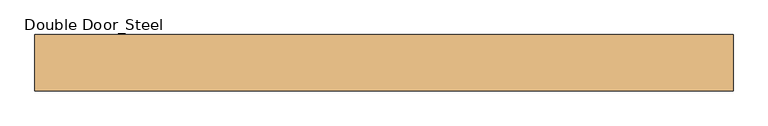
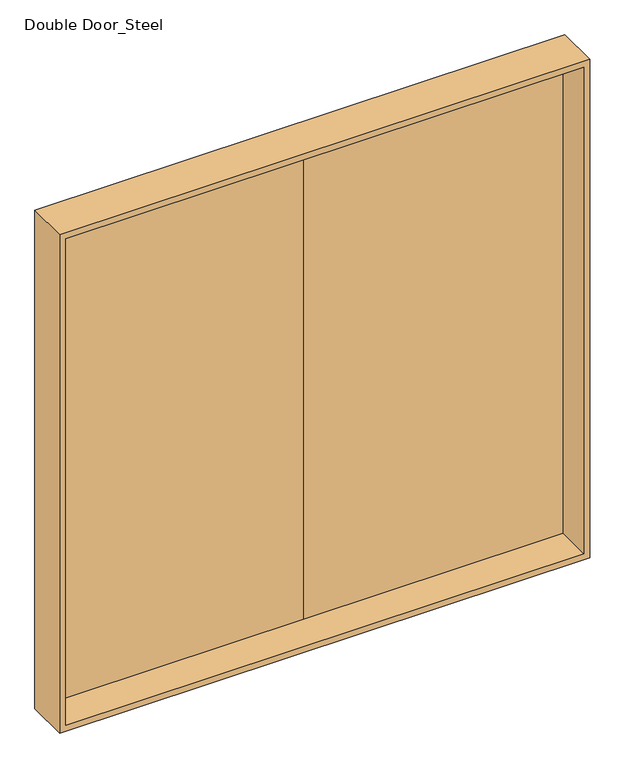
"""IFC4 building model written with IfcOpenShell, lengths in millimetres: door geometry, Double Door_Steel : H_DR_AR_B12_Double Door_Sliding_W3100xH3080_SD4."""

from ifc_helpers import new_model, si_unit, frame, origin, place, context, project, spatial, polyline, outline, extrude, faceted_brep, source, transform, mapped, element, save


def double_door_steel_99e35c84(model_context):
    return source(origin(), model_context, "Body", "SolidModel", [
        extrude(outline(polyline([(1530.0, 85.0), (0.0, 85.0), (0.0, 125.0), (1530.0, 125.0), (1530.0, 85.0)])), frame((0.0, 0.0, 20.0), z_axis=(0.0, 0.0, 1.0), x_axis=(1.0, 0.0, 0.0)), (0.0, 0.0, 1.0), 3040.0),
        extrude(outline(polyline([(0.0, 85.0), (-1530.0, 85.0), (-1530.0, 125.0), (0.0, 125.0), (0.0, 85.0)])), frame((0.0, 0.0, 20.0), z_axis=(0.0, 0.0, 1.0), x_axis=(1.0, 0.0, 0.0)), (0.0, 0.0, 1.0), 3040.0),
        faceted_brep([(1550.0, -125.0, 3080.0), (1550.0, 125.0, 3080.0), (-1550.0, 125.0, 3080.0), (-1550.0, -125.0, 3080.0), (1515.0, 85.0, 3045.0), (1515.0, -125.0, 3045.0), (-1515.0, -125.0, 3045.0), (-1515.0, 85.0, 3045.0), (1530.0, 125.0, 3060.0), (1530.0, 85.0, 3060.0), (-1530.0, 85.0, 3060.0), (-1530.0, 125.0, 3060.0), (-1550.0, 125.0, 0.0), (-1550.0, -125.0, 0.0), (-1515.0, -125.0, 35.0), (-1515.0, 85.0, 35.0), (-1530.0, 85.0, 20.0), (-1530.0, 125.0, 20.0), (1550.0, 125.0, 0.0), (1530.0, 125.0, 20.0), (1550.0, -125.0, 0.0), (1515.0, -125.0, 35.0), (1515.0, 85.0, 35.0), (1530.0, 85.0, 20.0)], [[[0, 1, 2, 3]], [[4, 5, 6, 7]], [[8, 9, 10, 11]], [[3, 2, 12, 13]], [[7, 6, 14, 15]], [[11, 10, 16, 17]], [[18, 12, 2, 1], [8, 11, 17, 19]], [[13, 12, 18, 20]], [[0, 3, 13, 20], [21, 14, 6, 5]], [[15, 14, 21, 22]], [[23, 16, 10, 9], [4, 7, 15, 22]], [[17, 16, 23, 19]], [[20, 18, 1, 0]], [[22, 21, 5, 4]], [[19, 23, 9, 8]]]),
    ])


if __name__ == "__main__":
    model = new_model("IFC4")
    model_context = context("Model", 3, world=origin())
    ifc_project = project(units=[si_unit("LENGTHUNIT", "METRE", prefix="MILLI")], contexts=[model_context])
    site = spatial("IfcSite", under=ifc_project)
    building = spatial("IfcBuilding", under=site)
    placement = place(None, origin())
    double_door_steel_shape = double_door_steel_99e35c84(model_context)
    element("IfcDoor", 1, ObjectType="Double Door_Steel : H_DR_AR_B12_Double Door_Sliding_W3100xH3080_SD4", at=placement, inside=building, context=model_context, shape_type="MappedRepresentation", body=[
        mapped(double_door_steel_shape, transform((0.0, 0.0, 0.0), x_axis=(1.0, 0.0, 0.0), y_axis=(0.0, 1.0, 0.0), z_axis=(0.0, 0.0, 1.0))),
    ])
    save(model, "model.ifc")

# Revit data of these elements
# Type "Double Door_Steel : H_DR_AR_B12_Double Door_Sliding_W3100xH3080_SD4"
#   Type Mark = "446"
#   프레임 = ""
#   철물 = ""
#   유리/마감 = ""
#   위치/개소 = ""
#   부호 = "1/SD"
#   문번호 = "4"
#   문기호 = "SD"
#   Analytic Construction = "<None>"
#   Height = 3080 mm
#   Width = 3100 mm
#   Define Thermal Properties by = 1
#   문 틀 = none
#   문 = none
#   Function = (empty or 0)
#   Assembly Code = ""
#   Wall Closure = (empty or 0)
